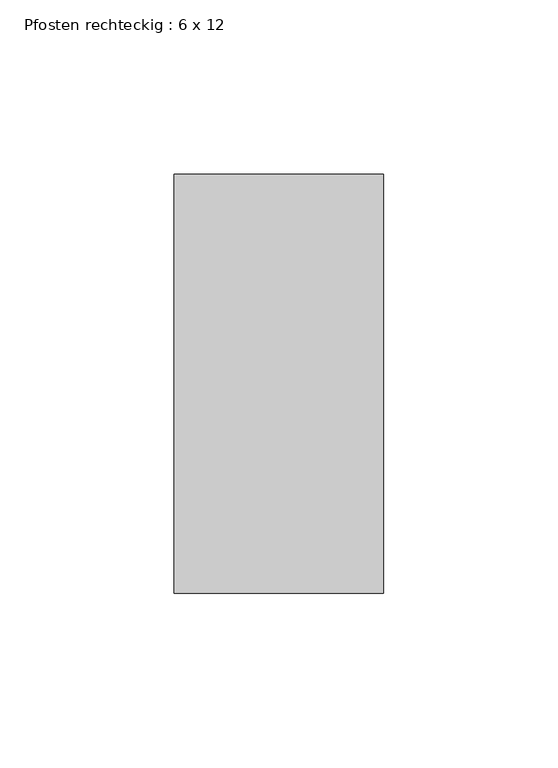
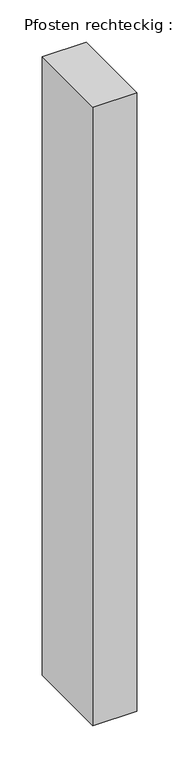
"""IFC4 building model written with IfcOpenShell, lengths in millimetres: member geometry, Pfosten rechteckig : 6 x 12."""

from ifc_helpers import new_model, si_unit, frame, origin, place, context, project, spatial, polyline, outline, extrude, source, transform, mapped, element, save


def pfosten_rechteckig_6_x_12_8f5ee4ad(model_context):
    return source(origin(), model_context, "Body", "SweptSolid", [
        extrude(outline(polyline([(0.0, 60.0), (0.0, -60.0), (-60.0, -60.0), (-60.0, 60.0), (0.0, 60.0)])), frame((0.0, 0.0, -895.0226945), z_axis=(0.0, 0.0, 1.0), x_axis=(1.0, 0.0, 0.0)), (0.0, 0.0, 1.0), 895.0226945),
    ])


if __name__ == "__main__":
    model = new_model("IFC4")
    model_context = context("Model", 3, world=origin())
    ifc_project = project(units=[si_unit("LENGTHUNIT", "METRE", prefix="MILLI")], contexts=[model_context])
    site = spatial("IfcSite", under=ifc_project)
    building = spatial("IfcBuilding", under=site)
    placement = place(None, origin())
    pfosten_rechteckig_6_x_12_shape = pfosten_rechteckig_6_x_12_8f5ee4ad(model_context)
    element("IfcMember", 1, ObjectType="Pfosten rechteckig : 6 x 12", at=placement, inside=building, context=model_context, shape_type="MappedRepresentation", body=[
        mapped(pfosten_rechteckig_6_x_12_shape, transform((0.0, 0.0, 0.0), x_axis=(1.0, 0.0, 0.0), y_axis=(0.0, 1.0, 0.0), z_axis=(0.0, 0.0, 1.0))),
    ])
    save(model, "model.ifc")

# Revit data of these elements
# Type "Pfosten rechteckig : 6 x 12"
#   built-in parameter 1007304 = 0.393701 (stored number, unit not read)
#   built-in parameter 1007301 = 0.0984252 (stored number, unit not read)
#   built-in parameter 1007300 = 0.0984252 (stored number, unit not read)
# Element 1 (IfcMember, "Pfosten rechteckig : 6 x 12")
#   Materials on its faces: "Metall - verzinkt"
# Materials
#   "Metall - verzinkt": class "Allgemeines", colour RGB 200 200 200, transparency 0, Cost = 0
